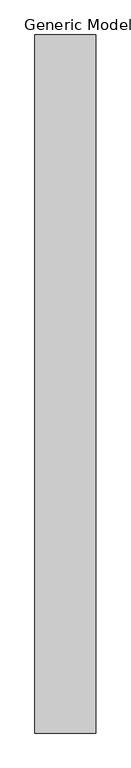
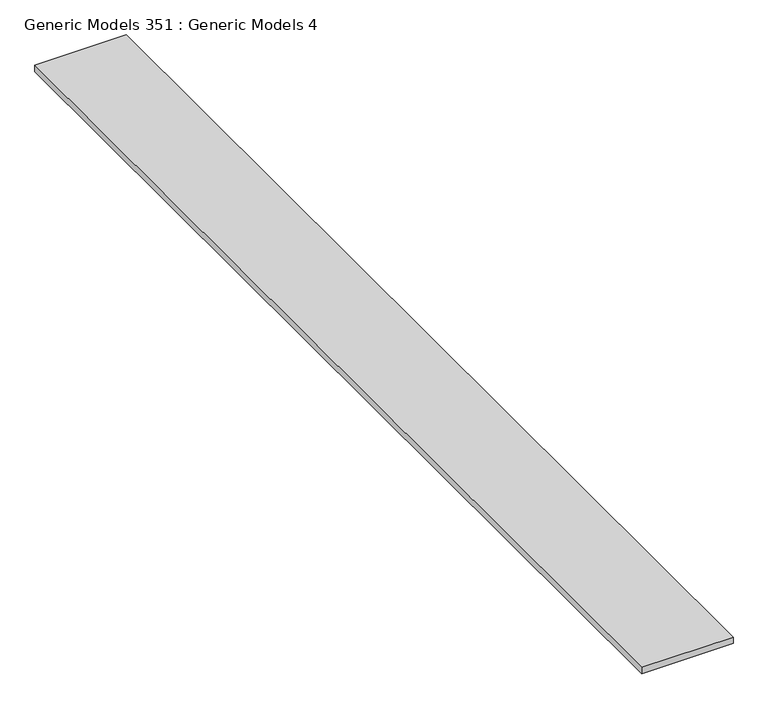
"""IFC4 building model written with IfcOpenShell, lengths in millimetres: proxy geometry, Generic Models 351 : Generic Models 4."""

from ifc_helpers import new_model, si_unit, frame, origin, place, context, project, spatial, polyline, outline, extrude, source, transform, mapped, element, save


def generic_models_351_generic_models_4_3c5a61cb(model_context):
    return source(origin(), model_context, "Body", "SweptSolid", [
        extrude(outline(polyline([(-6410.6047749, -6864.9230338), (-6967.8925756, -6864.9230338), (-6967.8925756, -464.1230338), (-6410.6047749, -464.1230338), (-6410.6047749, -6864.9230338)])), frame((0.0, 0.0, 129048.8656), z_axis=(0.0, 0.0, 1.0), x_axis=(1.0, 0.0, 0.0)), (0.0, 0.0, 1.0), 40.9598691),
    ])


if __name__ == "__main__":
    model = new_model("IFC4")
    model_context = context("Model", 3, world=origin())
    ifc_project = project(units=[si_unit("LENGTHUNIT", "METRE", prefix="MILLI")], contexts=[model_context])
    site = spatial("IfcSite", under=ifc_project)
    building = spatial("IfcBuilding", under=site)
    placement = place(None, origin())
    generic_models_351_generic_models_4_shape = generic_models_351_generic_models_4_3c5a61cb(model_context)
    element("IfcBuildingElementProxy", 1, Name="Generic Models 351 : Generic Models 4", ObjectType="Generic Models 351 : Generic Models 4", at=placement, inside=building, context=model_context, shape_type="MappedRepresentation", body=[
        mapped(generic_models_351_generic_models_4_shape, transform((0.0, 0.0, 0.0), x_axis=(1.0, 0.0, 0.0), y_axis=(0.0, 1.0, 0.0), z_axis=(0.0, 0.0, 1.0))),
    ])
    save(model, "model.ifc")

# Revit data of these elements
# Element 1 (IfcBuildingElementProxy, "Generic Models 351 : Generic Models 4")
#   Materials on its faces: "_BATT INSULATION (U-FACTOR = 0.065 MIN.) OVER CLASS II VAPOR RETARDER(TOWARD INTERIOR)"
# Materials
#   "_BATT INSULATION (U-FACTOR = 0.065 MIN.) OVER CLASS II VAPOR RETARDER(TOWARD INTERIOR)": class "Generic", colour RGB 200 166 247, transparency 0, Cost = 0
